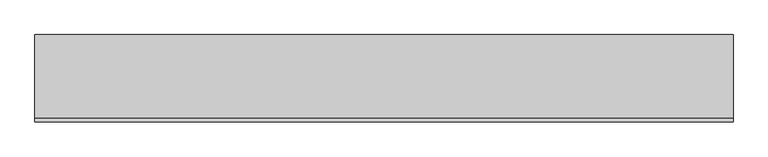
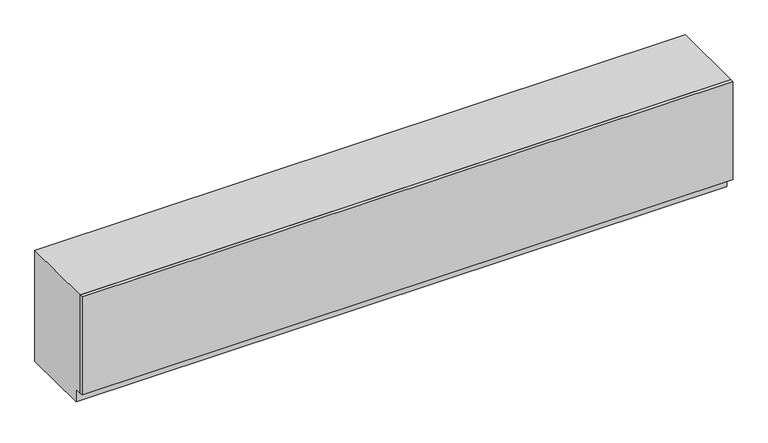
"""IFC4 building model written with IfcOpenShell, lengths in millimetres: furniture geometry, OD_CW_Base Cabinet : OD_CW_Base Cabinet."""

from ifc_helpers import new_model, si_unit, frame, origin, place, context, project, spatial, polyline, outline, extrude, source, transform, mapped, element, save


def furniture_f73364f5(model_context):
    return source(origin(), model_context, "Body", "SweptSolid", [
        extrude(outline(polyline([(18.7377049, 25.4), (4879.6627049, 25.4), (4879.6627049, 0.0), (18.7377049, 0.0), (18.7377049, 25.4)])), frame((0.0, 0.0, 101.6), z_axis=(0.0, 0.0, 1.0), x_axis=(1.0, 0.0, 0.0)), (0.0, 0.0, 1.0), 774.7),
        extrude(outline(polyline([(25.4, 876.3), (609.6, 876.3), (609.6, 0.0), (76.2, 0.0), (76.2, 101.6), (25.4, 101.6), (25.4, 876.3)])), frame((18.7377049, 0.0, 0.0), z_axis=(1.0, 0.0, 0.0), x_axis=(0.0, 1.0, 0.0)), (0.0, 0.0, 1.0), 4860.925),
    ])


if __name__ == "__main__":
    model = new_model("IFC4")
    model_context = context("Model", 3, world=origin())
    ifc_project = project(units=[si_unit("LENGTHUNIT", "METRE", prefix="MILLI")], contexts=[model_context])
    site = spatial("IfcSite", under=ifc_project)
    building = spatial("IfcBuilding", under=site)
    placement = place(None, origin())
    furniture_shape = furniture_f73364f5(model_context)
    element("IfcFurniture", 1, ObjectType="OD_CW_Base Cabinet : OD_CW_Base Cabinet", at=placement, inside=building, context=model_context, shape_type="MappedRepresentation", body=[
        mapped(furniture_shape, transform((0.0, 0.0, 0.0), x_axis=(1.0, 0.0, 0.0), y_axis=(0.0, 1.0, 0.0), z_axis=(0.0, 0.0, 1.0))),
    ])
    save(model, "model.ifc")

# Revit data of these elements
# Type "OD_CW_Base Cabinet : OD_CW_Base Cabinet"
#   OD_CW_Width [instance default] = 2' - 10"
#   OD_CW_Length [instance default] = 8' - 0"
#   OD_CW_Height [instance default] = 2' - 3"
#   Depth = 2' - 0"
#   Height = 3' - 0"
#   Width = 4' - 0"
#   OD_CW_Material_Front Panel [instance default] = none
#   OD_CW_Material_Body [instance default] = none
# Element 1 (IfcFurniture, "OD_CW_Base Cabinet : OD_CW_Base Cabinet")
#   OD_CW_Width = 2' - 0"
#   OD_CW_Length = 15' - 11 3/8"
#   OD_CW_Height = 2' - 10 1/2"
